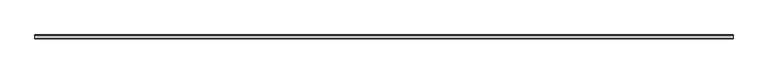
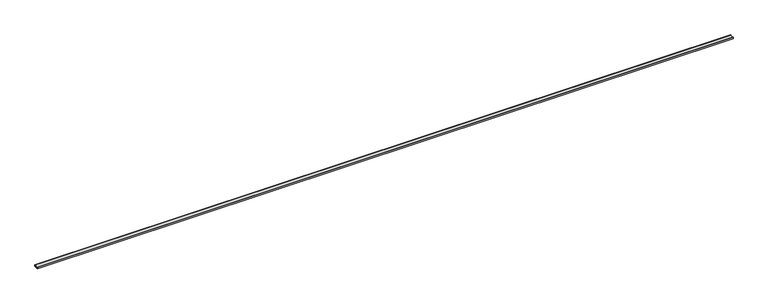
"""IFC4 building model written with IfcOpenShell, lengths in millimetres: proxy geometry, TSP LED Stip Light : TSP LED Stip Light."""

from ifc_helpers import new_model, si_unit, frame, origin, place, context, project, spatial, polyline, outline, extrude, source, transform, mapped, element, save


def electrical_fixtures_128b050d(model_context):
    return source(origin(), model_context, "Body", "SweptSolid", [
        extrude(outline(polyline([(-20.0, 0.0), (-20.0, 15.0), (-18.0, 15.0), (-18.0, 13.9588553), (-19.0050556, 13.9588553), (-19.0050556, 12.9537997), (-18.0, 12.9537997), (-18.0, 2.0), (18.0, 2.0), (18.0, 12.9537997), (19.0050556, 12.9537997), (19.0050556, 13.9588553), (18.0, 13.9588553), (18.0, 15.0), (20.0, 15.0), (20.0, 0.0), (-20.0, 0.0)])), frame((0.0, 0.0, 0.0), z_axis=(1.0, 0.0, 0.0), x_axis=(0.0, 1.0, 0.0)), (0.0, 0.0, 1.0), 6840.0465012),
        extrude(outline(polyline([(18.0, 13.9588553), (19.0050556, 13.9588553), (19.0050556, 12.9537997), (-19.0050556, 12.9537997), (-19.0050556, 13.9588553), (-18.0, 13.9588553), (-18.0, 15.0), (18.0, 15.0), (18.0, 13.9588553)])), frame((0.0, 0.0, 0.0), z_axis=(1.0, 0.0, 0.0), x_axis=(0.0, 1.0, 0.0)), (0.0, 0.0, 1.0), 6840.0465012),
    ])


if __name__ == "__main__":
    model = new_model("IFC4")
    model_context = context("Model", 3, world=origin())
    ifc_project = project(units=[si_unit("LENGTHUNIT", "METRE", prefix="MILLI")], contexts=[model_context])
    site = spatial("IfcSite", under=ifc_project)
    building = spatial("IfcBuilding", under=site)
    placement = place(None, origin())
    electrical_fixtures_shape = electrical_fixtures_128b050d(model_context)
    element("IfcBuildingElementProxy", 1, Name="TSP LED Stip Light : TSP LED Stip Light", ObjectType="TSP LED Stip Light : TSP LED Stip Light", at=placement, inside=building, context=model_context, shape_type="MappedRepresentation", body=[
        mapped(electrical_fixtures_shape, transform((0.0, 0.0, 0.0), x_axis=(1.0, 0.0, 0.0), y_axis=(0.0, 1.0, 0.0), z_axis=(0.0, 0.0, 1.0))),
    ])
    save(model, "model.ifc")

# Revit data of these elements
# Type "TSP LED Stip Light : TSP LED Stip Light"
#   Model = "TSP_ELECLEDSLINST"
#   built-in parameter 1001306 [instance default] = 5.24934 (stored number, unit not read)
#   Cable Length [instance default] = 1600 mm
#   Default Elevation = 0
# Element 1 (IfcBuildingElementProxy, "TSP LED Stip Light : TSP LED Stip Light")
#   built-in parameter 1001306 = 22.4411 (stored number, unit not read)
#   Cable Length = 6840.047 mm
#   Materials on its faces: "Aluminum, Anodized Silver", "Glass, White, High Luminance"
# Materials
#   "Aluminum, Anodized Silver": class "Metal", colour RGB 128 128 128, transparency 0, Description = "Anodized aluminum, silver", Cost = 0
#   "Glass, White, High Luminance": class "Glass", colour RGB 249 250 249, transparency 0.8, Description = "physical material", Cost = 0
